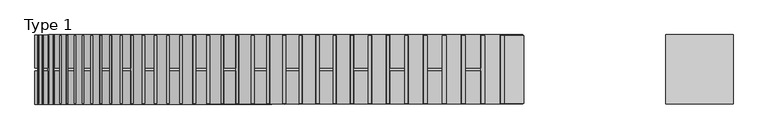
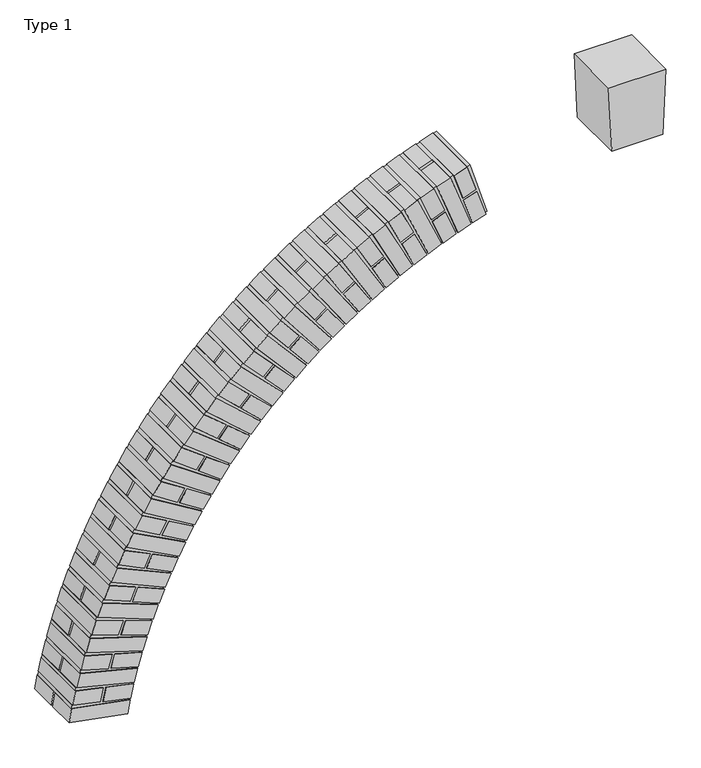
"""IFC4 building model written with IfcOpenShell, lengths in millimetres: proxy geometry, 00_GM_toog : Type 1."""

from ifc_helpers import new_model, si_unit, frame, origin, place, context, project, spatial, polyline, outline, extrude, source, transform, mapped, element, save


def type_1_a7bc3141(model_context):
    return source(origin(), model_context, "Body", "SweptSolid", [
        extrude(outline(polyline([(-139.1332824, -660.1921832), (-331.426292, -589.1357943), (-329.3635509, -583.5535983), (-240.0143287, -613.5107034), (-224.119862, -566.1043122), (-313.3029535, -536.2029076), (-311.2302503, -530.593752), (-115.9023342, -589.5306663), (-119.7774114, -601.0883632), (-214.5901938, -569.2994297), (-230.4846606, -616.7058209), (-135.6718782, -648.4947544), (-139.1332824, -660.1921832)])), frame((0.0, 2.5, 0.0), z_axis=(0.0, 1.0, 0.0), x_axis=(0.0, 0.0, 1.0)), (0.0, 0.0, 1.0), 205.0),
        extrude(outline(polyline([(0.0, -50.0), (0.0, 0.0), (210.0, 0.0), (210.0, -50.0), (0.0, -50.0)])), frame((-569.2994297, 210.0, -214.5901938), z_axis=(-0.3178893349961213, 0.0, 0.9481278240278174), x_axis=(0.0, -1.0, 0.0)), (0.0, 0.0, 1.0), 100.0),
        extrude(outline(polyline([(0.0, -50.0), (0.0, 0.0), (210.0, 0.0), (210.0, -50.0), (0.0, -50.0)])), frame((-534.3153787, 210.0, -318.9326444), z_axis=(-0.3178893349961213, 0.0, 0.9481278240278174), x_axis=(0.0, -1.0, 0.0)), (0.0, 0.0, 1.0), 100.0),
        extrude(outline(polyline([(210.0, -50.0), (110.0, -50.0), (110.0, 0.0), (210.0, 0.0), (210.0, -50.0)])), frame((-634.3036342, 0.0, -353.4456316), z_axis=(-0.3466140077500296, 0.0, 0.9380078515830571), x_axis=(0.0, 1.0, 0.0)), (0.0, 0.0, 1.0), 210.0),
        extrude(outline(polyline([(100.0, -50.0), (0.0, -50.0), (0.0, 0.0), (100.0, 0.0), (100.0, -50.0)])), frame((-634.3036342, 0.0, -353.4456316), z_axis=(-0.3466140077500296, 0.0, 0.9380078515830571), x_axis=(0.0, 1.0, 0.0)), (0.0, 0.0, 1.0), 210.0),
        extrude(outline(polyline([(-182.9035816, -776.5095671), (-370.5143948, -693.8790961), (-368.1156623, -688.4328225), (-280.7557912, -723.7735153), (-262.0049317, -677.4226224), (-349.2023711, -642.14764), (-346.7920539, -636.6750634), (-155.414188, -707.3932871), (-159.9856549, -718.6936531), (-252.6874407, -681.1919342), (-271.4383001, -727.5428271), (-178.7365144, -765.0445459), (-182.9035816, -776.5095671)])), frame((0.0, 2.5, 0.0), z_axis=(0.0, 1.0, 0.0), x_axis=(0.0, 0.0, 1.0)), (0.0, 0.0, 1.0), 205.0),
        extrude(outline(polyline([(0.0, -50.0), (0.0, 0.0), (210.0, 0.0), (210.0, -50.0), (0.0, -50.0)])), frame((-681.1919342, 210.0, -252.6874407), z_axis=(-0.37501718884823365, 0.0, 0.9270178574700534), x_axis=(0.0, -1.0, 0.0)), (0.0, 0.0, 1.0), 100.0),
        extrude(outline(polyline([(0.0, -50.0), (0.0, 0.0), (210.0, 0.0), (210.0, -50.0), (0.0, -50.0)])), frame((-639.9209035, 210.0, -354.7067175), z_axis=(-0.37501718884823365, 0.0, 0.9270178574700534), x_axis=(0.0, -1.0, 0.0)), (0.0, 0.0, 1.0), 100.0),
        extrude(outline(polyline([(210.0, -50.0), (110.0, -50.0), (110.0, 0.0), (210.0, 0.0), (210.0, -50.0)])), frame((-737.6227368, 0.0, -395.2424957), z_axis=(-0.40307253375327073, 0.0, 0.9151680351354708), x_axis=(0.0, 1.0, 0.0)), (0.0, 0.0, 1.0), 210.0),
        extrude(outline(polyline([(100.0, -50.0), (0.0, -50.0), (0.0, 0.0), (100.0, 0.0), (100.0, -50.0)])), frame((-737.6227368, 0.0, -395.2424957), z_axis=(-0.40307253375327073, 0.0, 0.9151680351354708), x_axis=(0.0, 1.0, 0.0)), (0.0, 0.0, 1.0), 210.0),
        extrude(outline(polyline([(-233.6735411, -889.9467043), (-415.9062676, -796.048646), (-413.1804412, -790.7584963), (-328.1339583, -831.3516903), (-306.5962573, -786.2282216), (-391.4846098, -745.7105041), (-388.7456188, -740.3948054), (-202.0276663, -822.6320289), (-207.2785664, -833.6331483), (-297.5255039, -790.5577463), (-319.0632049, -835.6812151), (-228.8162674, -878.7566171), (-233.6735411, -889.9467043)])), frame((0.0, 2.5, 0.0), z_axis=(0.0, 1.0, 0.0), x_axis=(0.0, 0.0, 1.0)), (0.0, 0.0, 1.0), 205.0),
        extrude(outline(polyline([(0.0, -50.0), (0.0, 0.0), (210.0, 0.0), (210.0, -50.0), (0.0, -50.0)])), frame((-790.5577463, 210.0, -297.5255039), z_axis=(-0.43075402055290246, 0.0, 0.9024693755344331), x_axis=(0.0, -1.0, 0.0)), (0.0, 0.0, 1.0), 100.0),
        extrude(outline(polyline([(0.0, -50.0), (0.0, 0.0), (210.0, 0.0), (210.0, -50.0), (0.0, -50.0)])), frame((-743.1528195, 210.0, -396.8431948), z_axis=(-0.43075402055290246, 0.0, 0.9024693755344331), x_axis=(0.0, -1.0, 0.0)), (0.0, 0.0, 1.0), 100.0),
        extrude(outline(polyline([(210.0, -50.0), (110.0, -50.0), (110.0, 0.0), (210.0, 0.0), (210.0, -50.0)])), frame((-838.2058326, 0.0, -443.2514078), z_axis=(-0.458035974096042, 0.0, 0.8889336569361574), x_axis=(0.0, 1.0, 0.0)), (0.0, 0.0, 1.0), 210.0),
        extrude(outline(polyline([(100.0, -50.0), (0.0, -50.0), (0.0, 0.0), (100.0, 0.0), (100.0, -50.0)])), frame((-838.2058326, 0.0, -443.2514078), z_axis=(-0.458035974096042, 0.0, 0.8889336569361574), x_axis=(0.0, 1.0, 0.0)), (0.0, 0.0, 1.0), 210.0),
        extrude(outline(polyline([(-291.2548438, -1000.0828313), (-467.4335419, -895.2654744), (-464.3907322, -890.151071), (-381.9730939, -935.8461971), (-357.7284394, -892.1175254), (-439.9928353, -846.5073621), (-436.9353302, -841.3682584), (-255.5698695, -934.8194455), (-261.4807258, -945.4805129), (-348.9380692, -896.9912039), (-373.1827237, -940.7198756), (-285.7253803, -989.2091846), (-291.2548438, -1000.0828313)])), frame((0.0, 2.5, 0.0), z_axis=(0.0, 1.0, 0.0), x_axis=(0.0, 0.0, 1.0)), (0.0, 0.0, 1.0), 205.0),
        extrude(outline(polyline([(0.0, -50.0), (0.0, 0.0), (210.0, 0.0), (210.0, -50.0), (0.0, -50.0)])), frame((-896.9912039, 210.0, -348.9380692), z_axis=(-0.4848930898069246, 0.0, 0.8745734339993948), x_axis=(0.0, -1.0, 0.0)), (0.0, 0.0, 1.0), 100.0),
        extrude(outline(polyline([(0.0, -50.0), (0.0, 0.0), (210.0, 0.0), (210.0, -50.0), (0.0, -50.0)])), frame((-843.6282164, 210.0, -445.1857828), z_axis=(-0.4848930898069246, 0.0, 0.8745734339993948), x_axis=(0.0, -1.0, 0.0)), (0.0, 0.0, 1.0), 100.0),
        extrude(outline(polyline([(210.0, -50.0), (110.0, -50.0), (110.0, 0.0), (210.0, 0.0), (210.0, -50.0)])), frame((-935.6798366, 0.0, -497.2942922), z_axis=(-0.5113004571556836, 0.0, 0.8594020261276959), x_axis=(0.0, 1.0, 0.0)), (0.0, 0.0, 1.0), 210.0),
        extrude(outline(polyline([(100.0, -50.0), (0.0, -50.0), (0.0, 0.0), (100.0, 0.0), (100.0, -50.0)])), frame((-935.6798366, 0.0, -497.2942922), z_axis=(-0.5113004571556836, 0.0, 0.8594020261276959), x_axis=(0.0, 1.0, 0.0)), (0.0, 0.0, 1.0), 210.0),
        extrude(outline(polyline([(-355.4339079, -1106.5094287), (-524.9050916, -991.1615642), (-521.5565851, -986.2418775), (-442.0734967, -1036.8694422), (-415.2118175, -994.6977669), (-494.5471198, -944.1643361), (-491.1824416, -939.2208894), (-315.8421974, -1043.5394089), (-322.3910854, -1053.82088), (-406.7344359, -1000.0975217), (-433.5961151, -1042.2691969), (-349.2527645, -1095.9925552), (-355.4339079, -1106.5094287)])), frame((0.0, 2.5, 0.0), z_axis=(0.0, 1.0, 0.0), x_axis=(0.0, 0.0, 1.0)), (0.0, 0.0, 1.0), 205.0),
        extrude(outline(polyline([(0.0, -50.0), (0.0, 0.0), (210.0, 0.0), (210.0, -50.0), (0.0, -50.0)])), frame((-1000.0975217, 210.0, -406.7344359), z_axis=(-0.5372335827633249, 0.0, 0.8434335051154191), x_axis=(0.0, -1.0, 0.0)), (0.0, 0.0, 1.0), 100.0),
        extrude(outline(polyline([(0.0, -50.0), (0.0, 0.0), (210.0, 0.0), (210.0, -50.0), (0.0, -50.0)])), frame((-940.9744086, 210.0, -499.5551681), z_axis=(-0.5372335827633249, 0.0, 0.8434335051154191), x_axis=(0.0, -1.0, 0.0)), (0.0, 0.0, 1.0), 100.0),
        extrude(outline(polyline([(210.0, -50.0), (110.0, -50.0), (110.0, 0.0), (210.0, 0.0), (210.0, -50.0)])), frame((-1029.683196, 0.0, -557.1706918), z_axis=(-0.562668413119899, 0.0, 0.8266826820958176), x_axis=(0.0, 1.0, 0.0)), (0.0, 0.0, 1.0), 210.0),
        extrude(outline(polyline([(100.0, -50.0), (0.0, -50.0), (0.0, 0.0), (100.0, 0.0), (100.0, -50.0)])), frame((-1029.683196, 0.0, -557.1706918), z_axis=(-0.562668413119899, 0.0, 0.8266826820958176), x_axis=(0.0, 1.0, 0.0)), (0.0, 0.0, 1.0), 210.0),
        extrude(outline(polyline([(-425.9726788, -1208.8317365), (-588.1077418, -1083.3812152), (-584.4659589, -1078.6744934), (-508.2122409, -1134.0467079), (-478.833173, -1093.5884532), (-554.9451095, -1038.3191945), (-551.2857383, -1033.5897414), (-382.6210868, -1148.3886526), (-389.7837151, -1158.252391), (-470.7002245, -1099.4942554), (-500.0792923, -1139.9525101), (-419.162783, -1198.7106457), (-425.9726788, -1208.8317365)])), frame((0.0, 2.5, 0.0), z_axis=(0.0, 1.0, 0.0), x_axis=(0.0, 0.0, 1.0)), (0.0, 0.0, 1.0), 205.0),
        extrude(outline(polyline([(0.0, -50.0), (0.0, 0.0), (210.0, 0.0), (210.0, -50.0), (0.0, -50.0)])), frame((-1099.4942554, 210.0, -470.7002245), z_axis=(-0.587581356894572, 0.0, 0.8091650938034423), x_axis=(0.0, -1.0, 0.0)), (0.0, 0.0, 1.0), 100.0),
        extrude(outline(polyline([(0.0, -50.0), (0.0, 0.0), (210.0, 0.0), (210.0, -50.0), (0.0, -50.0)])), frame((-1034.8303175, 210.0, -559.7496824), z_axis=(-0.587581356894572, 0.0, 0.8091650938034423), x_axis=(0.0, -1.0, 0.0)), (0.0, 0.0, 1.0), 100.0),
        extrude(outline(polyline([(210.0, -50.0), (110.0, -50.0), (110.0, 0.0), (210.0, 0.0), (210.0, -50.0)])), frame((-1119.8672315, 0.0, -622.6585117), z_axis=(-0.6119493068171298, 0.0, 0.7908969881634614), x_axis=(0.0, 1.0, 0.0)), (0.0, 0.0, 1.0), 210.0),
        extrude(outline(polyline([(100.0, -50.0), (0.0, -50.0), (0.0, 0.0), (100.0, 0.0), (100.0, -50.0)])), frame((-1119.8672315, 0.0, -622.6585117), z_axis=(-0.6119493068171298, 0.0, 0.7908969881634614), x_axis=(0.0, 1.0, 0.0)), (0.0, 0.0, 1.0), 210.0),
        extrude(outline(polyline([(-502.6095127, -1306.6702186), (-656.80706, -1171.5823645), (-652.8855088, -1167.1060659), (-580.1440032, -1227.0175422), (-548.3565201, -1188.4227768), (-620.9627746, -1128.6226962), (-617.022284, -1124.1247791), (-455.6588397, -1248.9782674), (-463.4086406, -1258.3876865), (-540.5981716, -1194.8127203), (-572.3856546, -1233.4074858), (-495.1961237, -1296.9824519), (-502.6095127, -1306.6702186)])), frame((0.0, 2.5, 0.0), z_axis=(0.0, 1.0, 0.0), x_axis=(0.0, 0.0, 1.0)), (0.0, 0.0, 1.0), 205.0),
        extrude(outline(polyline([(0.0, -50.0), (0.0, 0.0), (210.0, 0.0), (210.0, -50.0), (0.0, -50.0)])), frame((-1194.8127203, 210.0, -540.5981716), z_axis=(-0.6357496611103878, 0.0, 0.771895309221417), x_axis=(0.0, -1.0, 0.0)), (0.0, 0.0, 1.0), 100.0),
        extrude(outline(polyline([(0.0, -50.0), (0.0, 0.0), (210.0, 0.0), (210.0, -50.0), (0.0, -50.0)])), frame((-1124.8478107, 210.0, -625.546051), z_axis=(-0.6357496611103878, 0.0, 0.771895309221417), x_axis=(0.0, -1.0, 0.0)), (0.0, 0.0, 1.0), 100.0),
        extrude(outline(polyline([(210.0, -50.0), (110.0, -50.0), (110.0, 0.0), (210.0, 0.0), (210.0, -50.0)])), frame((-1205.8974304, 0.0, -693.514843), z_axis=(-0.658960344453872, 0.0, 0.752177681427224), x_axis=(0.0, 1.0, 0.0)), (0.0, 0.0, 1.0), 210.0),
        extrude(outline(polyline([(100.0, -50.0), (0.0, -50.0), (0.0, 0.0), (100.0, 0.0), (100.0, -50.0)])), frame((-1205.8974304, 0.0, -693.514843), z_axis=(-0.658960344453872, 0.0, 0.752177681427224), x_axis=(0.0, 1.0, 0.0)), (0.0, 0.0, 1.0), 210.0),
        extrude(outline(polyline([(-585.0601464, -1399.6619703), (-730.7482251, -1255.4378542), (-726.5614515, -1251.2085824), (-657.6019727, -1315.4370957), (-623.5239812, -1278.848976), (-692.355241, -1214.7398854), (-688.1482472, -1210.490188), (-534.684543, -1344.9351441), (-542.9927708, -1353.8553421), (-616.1690101, -1285.6993592), (-650.2470015, -1322.2874789), (-577.0707622, -1390.4434618), (-585.0601464, -1399.6619703)])), frame((0.0, 2.5, 0.0), z_axis=(0.0, 1.0, 0.0), x_axis=(0.0, 0.0, 1.0)), (0.0, 0.0, 1.0), 205.0),
        extrude(outline(polyline([(0.0, -50.0), (0.0, 0.0), (210.0, 0.0), (210.0, -50.0), (0.0, -50.0)])), frame((-1285.6993592, 210.0, -616.1690101), z_axis=(-0.6815598284590672, 0.0, 0.7317623932881814), x_axis=(0.0, -1.0, 0.0)), (0.0, 0.0, 1.0), 100.0),
        extrude(outline(polyline([(0.0, -50.0), (0.0, 0.0), (210.0, 0.0), (210.0, -50.0), (0.0, -50.0)])), frame((-1210.6929931, 210.0, -696.7002206), z_axis=(-0.6815598284590672, 0.0, 0.7317623932881814), x_axis=(0.0, -1.0, 0.0)), (0.0, 0.0, 1.0), 100.0),
        extrude(outline(polyline([(210.0, -50.0), (110.0, -50.0), (110.0, 0.0), (210.0, 0.0), (210.0, -50.0)])), frame((-1287.4546875, 0.0, -769.4768639), z_axis=(-0.7035271516375073, 0.0, 0.7106683804059498), x_axis=(0.0, 1.0, 0.0)), (0.0, 0.0, 1.0), 210.0),
        extrude(outline(polyline([(100.0, -50.0), (0.0, -50.0), (0.0, 0.0), (100.0, 0.0), (100.0, -50.0)])), frame((-1287.4546875, 0.0, -769.4768639), z_axis=(-0.7035271516375073, 0.0, 0.7106683804059498), x_axis=(0.0, 1.0, 0.0)), (0.0, 0.0, 1.0), 210.0),
        extrude(outline(polyline([(-673.0187522, -1487.4620645), (-809.6569728, -1334.6366457), (-805.2205066, -1330.670088), (-740.2988405, -1398.9774004), (-704.0567436, -1364.53164), (-768.8576982, -1296.3513341), (-764.3998058, -1292.3656196), (-619.4050728, -1435.9033572), (-628.2409103, -1444.3012472), (-697.1324311, -1371.8170533), (-733.374528, -1406.2628137), (-664.4830073, -1478.7470076), (-673.0187522, -1487.4620645)])), frame((0.0, 2.5, 0.0), z_axis=(0.0, 1.0, 0.0), x_axis=(0.0, 0.0, 1.0)), (0.0, 0.0, 1.0), 205.0),
        extrude(outline(polyline([(0.0, -99.9999999), (0.0, 0.0), (210.0, 0.0), (210.0, -99.9999999), (0.0, -99.9999999)])), frame((-1406.2628137, 210.0, -733.374528), z_axis=(0.6889152079134424, 0.0, 0.7248419388429304), x_axis=(0.0, -1.0, 0.0)), (0.0, 0.0, 1.0), 50.0),
        extrude(outline(polyline([(0.0, -100.0), (0.0, 0.0), (210.0, 0.0), (210.0, -100.0), (0.0, -100.0)])), frame((-1326.4932065, 210.0, -809.1903613), z_axis=(0.6889152079134424, 0.0, 0.7248419388429304), x_axis=(0.0, -1.0, 0.0)), (0.0, 0.0, 1.0), 50.0),
        extrude(outline(polyline([(0.0, -100.0), (0.0, 0.0), (209.9999999, 0.0), (209.9999999, -100.0), (0.0, -100.0)])), frame((-1364.2364889, 110.0, -850.2628142), z_axis=(0.6665230523277088, 0.0, 0.7454844201697004), x_axis=(-0.7454844201697004, 0.0, 0.6665230523277088)), (0.0, 0.0, 1.0), 50.0),
        extrude(outline(polyline([(0.0, -100.0), (0.0, 0.0), (209.9999999, 0.0), (209.9999999, -100.0), (0.0, -100.0)])), frame((-1364.2364889, 0.0, -850.2628142), z_axis=(0.6665230523277088, 0.0, 0.7454844201697004), x_axis=(-0.7454844201697004, 0.0, 0.6665230523277088)), (0.0, 0.0, 1.0), 50.0),
        extrude(outline(polyline([(-766.1590722, -1569.7448312), (-893.2406131, -1408.8849732), (-888.57091, -1405.1958423), (-827.9278656, -1477.3285868), (-789.6560932, -1445.1529526), (-850.1863815, -1373.1543275), (-845.4941258, -1369.4473798), (-709.5061817, -1521.5454855), (-718.8368549, -1529.3899178), (-783.1881232, -1452.8463729), (-821.4598957, -1485.022007), (-757.1086274, -1561.565552), (-766.1590722, -1569.7448312)])), frame((0.0, 2.5, 0.0), z_axis=(0.0, 1.0, 0.0), x_axis=(0.0, 0.0, 1.0)), (0.0, 0.0, 1.0), 205.0),
        extrude(outline(polyline([(0.0, -100.0000001), (0.0, 0.0), (210.0, 0.0), (210.0, -100.0000001), (0.0, -100.0000001)])), frame((-1485.022007, 210.0, -821.4598957), z_axis=(0.643512682835849, 0.0, 0.7654354492897545), x_axis=(0.0, -1.0, 0.0)), (0.0, 0.0, 1.0), 50.0),
        extrude(outline(polyline([(0.0, -100.0), (0.0, 0.0), (210.0, 0.0), (210.0, -100.0), (0.0, -100.0)])), frame((-1400.7850419, 210.0, -892.2791339), z_axis=(0.643512682835849, 0.0, 0.7654354492897545), x_axis=(0.0, -1.0, 0.0)), (0.0, 0.0, 1.0), 50.0),
        extrude(outline(polyline([(0.0, -100.0), (0.0, 0.0), (210.0, 0.0), (210.0, -100.0), (0.0, -100.0)])), frame((-1435.9580338, 110.0, -935.5730411), z_axis=(0.6199054420311093, 0.0, 0.7846765212112665), x_axis=(-0.7846765212112665, 0.0, 0.6199054420311093)), (0.0, 0.0, 1.0), 50.0),
        extrude(outline(polyline([(0.0, -100.0), (0.0, 0.0), (210.0, 0.0), (210.0, -100.0), (0.0, -100.0)])), frame((-1435.9580338, 0.0, -935.5730411), z_axis=(0.6199054420311093, 0.0, 0.7846765212112665), x_axis=(-0.7846765212112665, 0.0, 0.6199054420311093)), (0.0, 0.0, 1.0), 50.0),
        extrude(outline(polyline([(-864.1356281, -1646.2050652), (-981.1891156, -1477.9074329), (-976.3034966, -1474.5094128), (-920.1640125, -1550.200033), (-880.0045231, -1520.4138717), (-936.0396247, -1444.8639862), (-931.1304104, -1441.4495551), (-804.6536647, -1601.5438633), (-814.4445641, -1608.8057411), (-874.0168867, -1528.4867622), (-914.1763762, -1558.2729235), (-854.6040536, -1638.5919024), (-864.1356281, -1646.2050652)])), frame((0.0, 2.5, 0.0), z_axis=(0.0, 1.0, 0.0), x_axis=(0.0, 0.0, 1.0)), (0.0, 0.0, 1.0), 205.0),
        extrude(outline(polyline([(0.0, -100.0), (0.0, 0.0), (210.0, 0.0), (210.0, -100.0), (0.0, -100.0)])), frame((-1558.2729235, 210.0, -914.1763762), z_axis=(0.5957232261172445, 0.0, 0.8031897894423599), x_axis=(0.0, -1.0, 0.0)), (0.0, 0.0, 1.0), 50.0),
        extrude(outline(polyline([(0.0, -100.0), (0.0, 0.0), (210.0, 0.0), (210.0, -100.0), (0.0, -100.0)])), frame((-1469.881054, 210.0, -979.7363351), z_axis=(0.5957232261172445, 0.0, 0.8031897894423599), x_axis=(0.0, -1.0, 0.0)), (0.0, 0.0, 1.0), 50.0),
        extrude(outline(polyline([(0.0, -100.0), (0.0, 0.0), (210.0, 0.0), (210.0, -100.0), (0.0, -100.0)])), frame((-1502.3532911, 110.0, -1025.0911098), z_axis=(0.5709884645992758, 0.0, 0.8209580825441465), x_axis=(-0.8209580825441465, 0.0, 0.5709884645992758)), (0.0, 0.0, 1.0), 50.0),
        extrude(outline(polyline([(0.0, -100.0), (0.0, 0.0), (210.0, 0.0), (210.0, -100.0), (0.0, -100.0)])), frame((-1502.3532911, 0.0, -1025.0911098), z_axis=(0.5709884645992758, 0.0, 0.8209580825441465), x_axis=(-0.8209580825441465, 0.0, 0.5709884645992758)), (0.0, 0.0, 1.0), 50.0),
        extrude(outline(polyline([(-966.5850031, -1716.5591585), (-1073.1762598, -1541.4480054), (-1068.0928468, -1538.3537), (-1016.6651568, -1617.3214425), (-974.7669108, -1590.0352375), (-1026.0989792, -1511.214323), (-1020.9910156, -1508.1050735), (-904.4945987, -1675.6017587), (-914.7094076, -1682.2541462), (-969.2818175, -1598.4576542), (-1011.1800635, -1625.7438592), (-956.6076536, -1709.5403512), (-966.5850031, -1716.5591585)])), frame((0.0, 2.5, 0.0), z_axis=(0.0, 1.0, 0.0), x_axis=(0.0, 0.0, 1.0)), (0.0, 0.0, 1.0), 205.0),
        extrude(outline(polyline([(0.0, -100.0), (0.0, 0.0), (210.0, 0.0), (210.0, -100.0), (0.0, -100.0)])), frame((-1625.7438592, 210.0, -1011.1800635), z_axis=(0.5457240994797231, 0.0, 0.8379649200575435), x_axis=(0.0, -1.0, 0.0)), (0.0, 0.0, 1.0), 50.0),
        extrude(outline(polyline([(0.0, -100.0), (0.0, 0.0), (210.0, 0.0), (210.0, -100.0), (0.0, -100.0)])), frame((-1533.5249505, 210.0, -1071.2375667), z_axis=(0.5457240994797231, 0.0, 0.8379649200575435), x_axis=(0.0, -1.0, 0.0)), (0.0, 0.0, 1.0), 50.0),
        extrude(outline(polyline([(0.0, -100.0), (0.0, 0.0), (210.0, 0.0), (210.0, -100.0), (0.0, -100.0)])), frame((-1563.1759859, 110.0, -1118.4849779), z_axis=(0.5199535639793587, 0.0, 0.854194527789287), x_axis=(-0.854194527789287, 0.0, 0.5199535639793587)), (0.0, 0.0, 1.0), 50.0),
        extrude(outline(polyline([(0.0, -100.0), (0.0, 0.0), (210.0, 0.0), (210.0, -100.0), (0.0, -100.0)])), frame((-1563.1759859, 0.0, -1118.4849779), z_axis=(0.5199535639793587, 0.0, 0.854194527789287), x_axis=(-0.854194527789287, 0.0, 0.5199535639793587)), (0.0, 0.0, 1.0), 50.0),
        extrude(outline(polyline([(-1073.1271897, -1780.5461522), (-1168.8608449, -1599.2710044), (-1163.5984934, -1596.4918913), (-1117.0733542, -1678.4438472), (-1073.5917616, -1653.7588091), (-1120.0303947, -1571.9592298), (-1114.7426284, -1569.1666948), (-1008.6586513, -1743.4444745), (-1019.2594808, -1749.4626965), (-1068.6295568, -1662.4995113), (-1112.1111495, -1687.1845493), (-1062.7410734, -1774.1477346), (-1073.1271897, -1780.5461522)])), frame((0.0, 2.5, 0.0), z_axis=(0.0, 1.0, 0.0), x_axis=(0.0, 0.0, 1.0)), (0.0, 0.0, 1.0), 205.0),
        extrude(outline(polyline([(0.0, -100.0000001), (0.0, 0.0), (210.0, 0.0), (210.0, -100.0000001), (0.0, -100.0000001)])), frame((-1687.1845493, 210.0, -1112.1111495), z_axis=(0.4937007608024789, 0.0, 0.8696318524427756), x_axis=(0.0, -1.0, 0.0)), (0.0, 0.0, 1.0), 50.0),
        extrude(outline(polyline([(0.0, -100.0000001), (0.0, 0.0), (210.0, 0.0), (210.0, -100.0000001), (0.0, -100.0000001)])), frame((-1591.4806619, 210.0, -1166.4434303), z_axis=(0.4937007608024789, 0.0, 0.8696318524427756), x_axis=(0.0, -1.0, 0.0)), (0.0, 0.0, 1.0), 50.0),
        extrude(outline(polyline([(0.0, -100.0), (0.0, 0.0), (210.0, 0.0), (210.0, -100.0), (0.0, -100.0)])), frame((-1618.2005133, 110.0, -1215.4082269), z_axis=(0.46699003996658267, 0.0, 0.8842625755803587), x_axis=(-0.8842625755803587, 0.0, 0.46699003996658267)), (0.0, 0.0, 1.0), 50.0),
        extrude(outline(polyline([(0.0, -100.0), (0.0, 0.0), (210.0, 0.0), (210.0, -100.0), (0.0, -100.0)])), frame((-1618.2005133, 0.0, -1215.4082269), z_axis=(0.46699003996658267, 0.0, 0.8842625755803587), x_axis=(-0.8842625755803587, 0.0, 0.46699003996658267)), (0.0, 0.0, 1.0), 50.0),
        extrude(outline(polyline([(-1183.3669992, -1837.9287043), (-1267.8879555, -1651.1619516), (-1262.4661848, -1648.7083391), (-1221.0161685, -1733.3405303), (-1176.1125121, -1711.3482215), (-1217.4854587, -1626.8733903), (-1212.0375032, -1624.4079279), (-1116.7594551, -1804.8203672), (-1127.7069842, -1810.1821007), (-1171.6916018, -1720.374788), (-1216.5952582, -1742.3670968), (-1172.6106405, -1832.1744095), (-1183.3669992, -1837.9287043)])), frame((0.0, 2.5, 0.0), z_axis=(0.0, 1.0, 0.0), x_axis=(0.0, 0.0, 1.0)), (0.0, 0.0, 1.0), 205.0),
        extrude(outline(polyline([(0.0, -100.0), (0.0, 0.0), (210.0, 0.0), (210.0, -100.0), (0.0, -100.0)])), frame((-1742.3670968, 210.0, -1216.5952582), z_axis=(0.43984617621729644, 0.0, 0.8980731269039415), x_axis=(0.0, -1.0, 0.0)), (0.0, 0.0, 1.0), 50.0),
        extrude(outline(polyline([(0.0, -100.0), (0.0, 0.0), (210.0, 0.0), (210.0, -100.0), (0.0, -100.0)])), frame((-1643.5332176, 210.0, -1265.0007861), z_axis=(0.43984617621729644, 0.0, 0.8980731269039415), x_axis=(0.0, -1.0, 0.0)), (0.0, 0.0, 1.0), 50.0),
        extrude(outline(polyline([(0.0, -100.0), (0.0, 0.0), (210.0, 0.0), (210.0, -100.0), (0.0, -100.0)])), frame((-1667.2227752, 110.0, -1315.5013467), z_axis=(0.412294346049213, 0.0, 0.9110506968417574), x_axis=(-0.9110506968417574, 0.0, 0.412294346049213)), (0.0, 0.0, 1.0), 50.0),
        extrude(outline(polyline([(0.0, -100.0), (0.0, 0.0), (210.0, 0.0), (210.0, -100.0), (0.0, -100.0)])), frame((-1667.2227752, 0.0, -1315.5013467), z_axis=(0.412294346049213, 0.0, 0.9110506968417574), x_axis=(-0.9110506968417574, 0.0, 0.412294346049213)), (0.0, 0.0, 1.0), 50.0),
        extrude(outline(polyline([(-1296.8955277, -1888.4939701), (-1369.8902781, -1696.928372), (-1364.3291986, -1694.809361), (-1328.1080526, -1781.807868), (-1281.9488902, -1762.5898628), (-1318.1026887, -1675.7531156), (-1312.5147517, -1673.6238707), (-1228.39604, -1859.5017797), (-1239.649662, -1864.1871369), (-1278.0856724, -1771.8688121), (-1324.2448348, -1791.0868173), (-1285.8088244, -1883.4051422), (-1296.8955277, -1888.4939701)])), frame((0.0, 2.5, 0.0), z_axis=(0.0, 1.0, 0.0), x_axis=(0.0, 0.0, 1.0)), (0.0, 0.0, 1.0), 205.0),
        extrude(outline(polyline([(0.0, -100.0), (0.0, 0.0), (210.0, 0.0), (210.0, -100.0), (0.0, -100.0)])), frame((-1791.0868173, 210.0, -1324.2448348), z_axis=(0.384360104354249, 0.0, 0.9231832484294713), x_axis=(0.0, -1.0, 0.0)), (0.0, 0.0, 1.0), 50.0),
        extrude(outline(polyline([(0.0, -99.9999999), (0.0, 0.0), (210.0, 0.0), (210.0, -99.9999999), (0.0, -99.9999999)])), frame((-1689.4895432, 210.0, -1366.544063), z_axis=(0.384360104354249, 0.0, 0.9231832484294713), x_axis=(0.0, -1.0, 0.0)), (0.0, 0.0, 1.0), 50.0),
        extrude(outline(polyline([(0.0, -100.0), (0.0, 0.0), (210.0, 0.0), (210.0, -100.0), (0.0, -100.0)])), frame((-1710.0609371, 110.0, -1418.3930699), z_axis=(0.3560693607188781, 0.0, 0.9344595284747487), x_axis=(-0.9344595284747487, 0.0, 0.3560693607188781)), (0.0, 0.0, 1.0), 50.0),
        extrude(outline(polyline([(0.0, -100.0), (0.0, 0.0), (210.0, 0.0), (210.0, -100.0), (0.0, -100.0)])), frame((-1710.0609371, 0.0, -1418.3930699), z_axis=(0.3560693607188781, 0.0, 0.9344595284747487), x_axis=(-0.9344595284747487, 0.0, 0.3560693607188781)), (0.0, 0.0, 1.0), 50.0),
        extrude(outline(polyline([(-1413.2916726, -1932.0543918), (-1474.4894633, -1736.4005077), (-1468.8097024, -1734.6239581), (-1437.9517789, -1823.6660841), (-1390.708325, -1807.2936664), (-1421.5088731, -1718.4171), (-1415.8016814, -1716.6319704), (-1343.1543211, -1907.2858866), (-1354.6722938, -1911.2774885), (-1387.4171293, -1816.7905807), (-1434.6605832, -1833.1629985), (-1401.9157477, -1927.6499063), (-1413.2916726, -1932.0543918)])), frame((0.0, 2.5, 0.0), z_axis=(0.0, 1.0, 0.0), x_axis=(0.0, 0.0, 1.0)), (0.0, 0.0, 1.0), 205.0),
        extrude(outline(polyline([(0.0, -100.0), (0.0, 0.0), (210.0, 0.0), (210.0, -100.0), (0.0, -100.0)])), frame((-1833.1629985, 210.0, -1434.6605832), z_axis=(0.3274483553925278, 0.0, 0.9448690779947923), x_axis=(0.0, -1.0, 0.0)), (0.0, 0.0, 1.0), 50.0),
        extrude(outline(polyline([(0.0, -100.0), (0.0, 0.0), (210.0, 0.0), (210.0, -100.0), (0.0, -100.0)])), frame((-1729.1791763, 210.0, -1470.6966144), z_axis=(0.3274483553925278, 0.0, 0.9448690779947923), x_axis=(0.0, -1.0, 0.0)), (0.0, 0.0, 1.0), 50.0),
        extrude(outline(polyline([(0.0, -100.0), (0.0, 0.0), (210.0, 0.0), (210.0, -100.0), (0.0, -100.0)])), frame((-1746.5561027, 110.0, -1523.701748), z_axis=(0.29852363494913453, 0.0, 0.9544022419172934), x_axis=(-0.9544022419172934, 0.0, 0.29852363494913453)), (0.0, 0.0, 1.0), 50.0),
        extrude(outline(polyline([(0.0, -100.0), (0.0, 0.0), (210.0, 0.0), (210.0, -100.0), (0.0, -100.0)])), frame((-1746.5561027, 0.0, -1523.701748), z_axis=(0.29852363494913453, 0.0, 0.9544022419172934), x_axis=(-0.9544022419172934, 0.0, 0.29852363494913453)), (0.0, 0.0, 1.0), 50.0),
        extrude(outline(polyline([(-1532.1236947, -1968.4483941), (-1581.2975296, -1769.4319478), (-1575.5201547, -1768.0044492), (-1550.1399126, -1858.7599172), (-1501.9874037, -1845.2938158), (-1527.3204552, -1754.7070932), (-1521.5151782, -1753.2727005), (-1460.6086345, -1947.9954461), (-1472.3482352, -1951.2784869), (-1499.2804379, -1854.9734691), (-1547.4329468, -1868.4395705), (-1520.5007441, -1964.7445883), (-1532.1236947, -1968.4483941)])), frame((0.0, 2.5, 0.0), z_axis=(0.0, 1.0, 0.0), x_axis=(0.0, 0.0, 1.0)), (0.0, 0.0, 1.0), 205.0),
        extrude(outline(polyline([(0.0, -100.0), (0.0, 0.0), (210.0, 0.0), (210.0, -100.0), (0.0, -100.0)])), frame((-1868.4395705, 210.0, -1547.4329468), z_axis=(0.2693220276647166, 0.0, 0.9630501780356856), x_axis=(0.0, -1.0, 0.0)), (0.0, 0.0, 1.0), 50.0),
        extrude(outline(polyline([(0.0, -100.0), (0.0, 0.0), (210.0, 0.0), (210.0, -100.0), (0.0, -100.0)])), frame((-1762.4548994, 210.0, -1577.0721153), z_axis=(0.2693220276647166, 0.0, 0.9630501780356856), x_axis=(0.0, -1.0, 0.0)), (0.0, 0.0, 1.0), 50.0),
        extrude(outline(polyline([(0.0, -100.0), (0.0, 0.0), (210.0, 0.0), (210.0, -100.0), (0.0, -100.0)])), frame((-1776.5729033, 110.0, -1631.0367679), z_axis=(0.23987061863352377, 0.0, 0.9708048652104967), x_axis=(-0.9708048652104967, 0.0, 0.23987061863352377)), (0.0, 0.0, 1.0), 50.0),
        extrude(outline(polyline([(0.0, -100.0), (0.0, 0.0), (210.0, 0.0), (210.0, -100.0), (0.0, -100.0)])), frame((-1776.5729033, 0.0, -1631.0367679), z_axis=(0.23987061863352377, 0.0, 0.9708048652104967), x_axis=(-0.9708048652104967, 0.0, 0.23987061863352377)), (0.0, 0.0, 1.0), 50.0),
        extrude(outline(polyline([(-1652.9508197, -1997.5409836), (-1689.9183019, -1795.9001713), (-1684.0647426, -1794.8270187), (-1664.2563229, -1886.9591964), (-1615.3733674, -1876.4493601), (-1635.1449565, -1784.4884876), (-1629.2631271, -1783.4101522), (-1580.323316, -1981.4794572), (-1592.2409998, -1984.0417594), (-1613.2606723, -1886.2758483), (-1662.1436278, -1896.7856846), (-1641.1239554, -1994.5515957), (-1652.9508197, -1997.5409836)])), frame((0.0, 2.5, 0.0), z_axis=(0.0, 1.0, 0.0), x_axis=(0.0, 0.0, 1.0)), (0.0, 0.0, 1.0), 205.0),
        extrude(outline(polyline([(0.0, -100.0), (0.0, 0.0), (210.0, 0.0), (210.0, -100.0), (0.0, -100.0)])), frame((-1896.7856846, 210.0, -1662.1436278), z_axis=(0.2101967246461282, 0.0, 0.9776591108090998), x_axis=(0.0, -1.0, 0.0)), (0.0, 0.0, 1.0), 50.0),
        extrude(outline(polyline([(0.0, -100.0), (0.0, 0.0), (210.0, 0.0), (210.0, -100.0), (0.0, -100.0)])), frame((-1789.1932853, 210.0, -1685.2759954), z_axis=(0.2101967246461282, 0.0, 0.9776591108090998), x_axis=(0.0, -1.0, 0.0)), (0.0, 0.0, 1.0), 50.0),
        extrude(outline(polyline([(0.0, -100.0), (0.0, 0.0), (210.0, 0.0), (210.0, -100.0), (0.0, -100.0)])), frame((-1800.0, 110.0, -1740.0), z_axis=(0.18032786885245566, 0.0, 0.9836065573770498), x_axis=(-0.9836065573770498, 0.0, 0.18032786885245566)), (0.0, 0.0, 1.0), 50.0),
        extrude(outline(polyline([(0.0, -100.0), (0.0, 0.0), (210.0, 0.0), (210.0, -100.0), (0.0, -100.0)])), frame((-1800.0, 0.0, -1740.0), z_axis=(0.18032786885245566, 0.0, 0.9836065573770498), x_axis=(-0.9836065573770498, 0.0, 0.18032786885245566)), (0.0, 0.0, 1.0), 50.0),
        extrude(outline(polyline([(0.0, 101.4705882), (0.0, -101.4705882), (-240.0, -89.7058824), (-240.0, 89.7058824), (0.0, 101.4705882)])), frame((0.0, 0.0, 0.0), z_axis=(0.0, 1.0, 0.0), x_axis=(0.0, 0.0, 1.0)), (0.0, 0.0, 1.0), 210.0),
    ])


if __name__ == "__main__":
    model = new_model("IFC4")
    model_context = context("Model", 3, world=origin())
    ifc_project = project(units=[si_unit("LENGTHUNIT", "METRE", prefix="MILLI")], contexts=[model_context])
    site = spatial("IfcSite", under=ifc_project)
    building = spatial("IfcBuilding", under=site)
    placement = place(None, origin())
    type_1_shape = type_1_a7bc3141(model_context)
    element("IfcBuildingElementProxy", 1, Name="00_GM_toog : Type 1", ObjectType="00_GM_toog : Type 1", at=placement, inside=building, context=model_context, shape_type="MappedRepresentation", body=[
        mapped(type_1_shape, transform((0.0, 0.0, 0.0), x_axis=(1.0, 0.0, 0.0), y_axis=(0.0, 1.0, 0.0), z_axis=(0.0, 0.0, 1.0))),
    ])
    save(model, "model.ifc")

# Revit data of these elements
# Type "00_GM_toog : Type 1"
#   straal_hart_rollaag [instance default] = 1935 mm
#   straal_buitenlijn [instance default] = 2040 mm
#   straal [instance default] = 1830 mm
#   stootvoegbreedte_onderzijde [instance default] = 5 mm
#   offset [instance default] = -2070 mm
#   kop_voeg [instance default] = 55 mm
#   hoek_sluitsteen_half [instance default] = 2.80637°
#   hoek_kop [instance default] = 1.72149°
#   halve_breedte_tov_balk [instance default] = 200 mm
#   half_b [instance default] = 1800 mm
#   h_toog [instance default] = 1500 mm
#   h_steen [instance default] = 210 mm
#   h_sluitsteen [instance default] = 240 mm
#   h_kop [instance default] = 50 mm
#   dekdikte [instance default] = 240 mm
#   breedte [instance default] = 4000 mm
#   b_sluitsteen_bovenzijde [instance default] = 200 mm
#   apothema [instance default] = 330 mm
#   aantal_strekken [instance default] = 14
#   materiaal_voeg [instance default] = none
#   materiaal_strek [instance default] = none
#   materiaal_sluitsteen [instance default] = none
#   materiaal_koppen [instance default] = none
#   Default Elevation = 0
